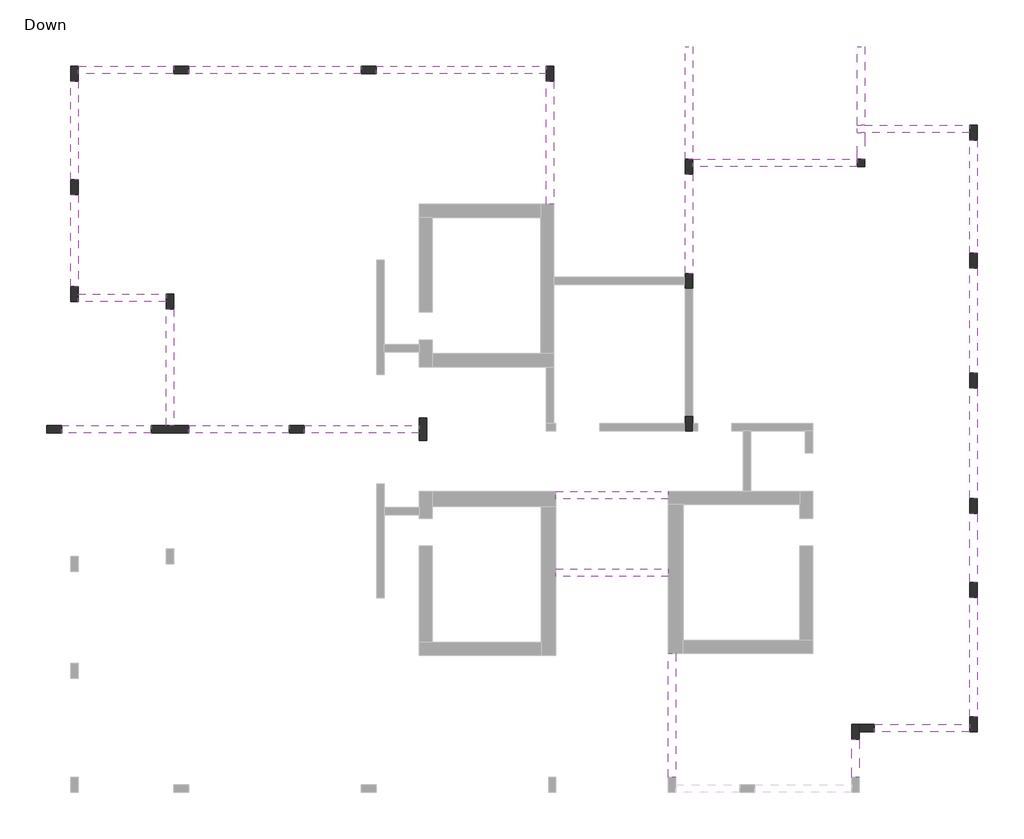
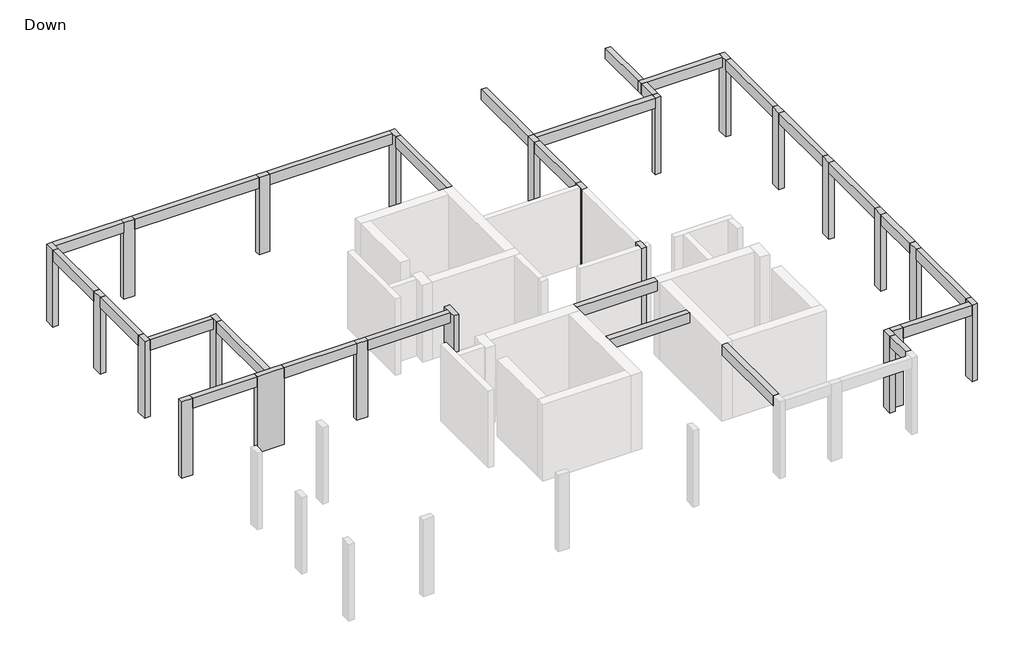
# One storey, part 2 of 2: 27 beams, 23 columns.
"""IFC4 building model written with IfcOpenShell, lengths in millimetres."""

from ifc_helpers import new_model, si_unit, frame, origin, origin_with_axes, place, context, project, spatial, polyline, outline, extrude, faceted_brep, element, save

model = new_model("IFC4")

# Units and contexts
model_context = context("Model", 3, world=origin())
ifc_project = project(units=[si_unit("LENGTHUNIT", "METRE", prefix="MILLI")], contexts=[model_context])

# Site, building, storey
site = spatial("IfcSite", under=ifc_project)
building = spatial("IfcBuilding", under=site)
storey = spatial("IfcBuildingStorey", under=building, Name="Down", Elevation=0.0)

# Beams
placement = place(None, origin())
element("IfcBeam", 1, ObjectType="Concrete Rectengular Beam : 20/40", at=placement, inside=storey, context=model_context, shape_type="SweptSolid", body=[
    extrude(outline(polyline([(-8952.4882749, 10699.8774677), (-8952.4882749, 10899.8774677), (-4346.8056177, 10899.8774677), (-4346.8056177, 10699.8774677), (-8952.4882749, 10699.8774677)])), frame((0.0, 0.0, 2600.0), z_axis=(0.0, 0.0, 1.0), x_axis=(1.0, 0.0, 0.0)), (0.0, 0.0, 1.0), 400.0),
])
element("IfcBeam", 2, ObjectType="Concrete Rectengular Beam : 20/40", at=placement, inside=storey, context=model_context, shape_type="Brep", body=[
    faceted_brep([(-11896.6244933, 10899.8774677, 3000.0), (-11896.6244933, 10699.8774677, 3000.0), (-9352.4882749, 10699.8774677, 3000.0), (-9352.4882749, 10899.8774677, 3000.0), (-11896.6244933, 10899.8774677, 2600.0), (-9352.4882749, 10899.8774677, 2600.0), (-11896.6244933, 10699.8774677, 2600.0), (-9352.4882749, 10699.8774677, 2600.0), (-11896.6244933, 10699.8774677, 2780.0)], [[[0, 1, 2, 3]], [[4, 0, 3, 5]], [[6, 4, 5, 7]], [[1, 8, 6, 7, 2]], [[1, 0, 4, 6, 8]], [[3, 2, 7, 5]]]),
])
element("IfcBeam", 3, ObjectType="Concrete Rectengular Beam : 20/40", at=placement, inside=storey, context=model_context, shape_type="SweptSolid", body=[
    extrude(outline(polyline([(-12096.6244933, 10499.8774677), (-11896.6244933, 10499.8774677), (-11896.6244933, 7862.3669988), (-12096.6244933, 7862.3669988), (-12096.6244933, 10499.8774677)])), frame((0.0, 0.0, 2600.0), z_axis=(0.0, 0.0, 1.0), x_axis=(1.0, 0.0, 0.0)), (0.0, 0.0, 1.0), 400.0),
])
element("IfcBeam", 4, ObjectType="Concrete Rectengular Beam : 20/40", at=placement, inside=storey, context=model_context, shape_type="SweptSolid", body=[
    extrude(outline(polyline([(-12096.6244933, 7462.3669988), (-11896.6244933, 7462.3669988), (-11896.6244933, 5012.2302086), (-12096.6244933, 5012.2302086), (-12096.6244933, 7462.3669988)])), frame((0.0, 0.0, 2600.0), z_axis=(0.0, 0.0, 1.0), x_axis=(1.0, 0.0, 0.0)), (0.0, 0.0, 1.0), 400.0),
])
element("IfcBeam", 5, ObjectType="Concrete Rectengular Beam : 20/40", at=placement, inside=storey, context=model_context, shape_type="Brep", body=[
    faceted_brep([(-9554.6843469, 4790.1128337, 3000.0), (-11896.6244933, 4790.1128337, 3000.0), (-11896.6244933, 4612.2302086, 3000.0), (-9554.6843469, 4612.2302086, 3000.0), (-9554.6843469, 4812.2302086, 2780.0), (-9554.6843469, 4812.2302086, 2600.0), (-11896.6244933, 4812.2302086, 2600.0), (-11896.6244933, 4812.2302086, 2780.0), (-9554.6843469, 4612.2302086, 2600.0), (-11896.6244933, 4612.2302086, 2600.0), (-9554.6843469, 4612.2302086, 2780.0), (-9554.6843469, 4790.1128337, 2780.0), (-11896.6244933, 4790.1128337, 2780.0)], [[[0, 1, 2, 3]], [[4, 5, 6, 7]], [[5, 8, 9, 6]], [[8, 10, 3, 2, 9]], [[8, 5, 4, 11, 0, 3, 10]], [[12, 11, 4, 7]], [[11, 12, 1, 0]], [[2, 1, 12, 7, 6, 9]]]),
])
element("IfcBeam", 6, ObjectType="Concrete Rectengular Beam : 20/40", at=placement, inside=storey, context=model_context, shape_type="Brep", body=[
    faceted_brep([(-9354.6843469, 4412.2302086, 3000.0), (-9554.6843469, 4412.2302086, 3000.0), (-9554.6843469, 1306.8737687, 3000.0), (-9354.6843469, 1306.8737687, 3000.0), (-9554.6843469, 4412.2302086, 2600.0), (-9554.6843469, 1306.8737687, 2600.0), (-9554.6843469, 1306.8737687, 2780.0), (-9354.6843469, 4412.2302086, 2600.0), (-9354.6843469, 1306.8737687, 2600.0), (-9354.6843469, 1306.8737687, 2780.0), (-9354.6843469, 4412.2302086, 2780.0)], [[[0, 1, 2, 3]], [[1, 4, 5, 6, 2]], [[4, 7, 8, 5]], [[0, 3, 9, 8, 7, 10]], [[1, 0, 10, 7, 4]], [[3, 2, 6, 5, 8, 9]]]),
])
element("IfcBeam", 7, ObjectType="Concrete Rectengular Beam : 20/40", at=placement, inside=storey, context=model_context, shape_type="SweptSolid", body=[
    extrude(outline(polyline([(-12343.1090323, 1106.8737687), (-12343.1090323, 1306.8737687), (-9954.6843469, 1306.8737687), (-9954.6843469, 1106.8737687), (-12343.1090323, 1106.8737687)])), frame((0.0, 0.0, 2600.0), z_axis=(0.0, 0.0, 1.0), x_axis=(1.0, 0.0, 0.0)), (0.0, 0.0, 1.0), 400.0),
])
element("IfcBeam", 8, ObjectType="Concrete Rectengular Beam : 20/40", at=placement, inside=storey, context=model_context, shape_type="SweptSolid", body=[
    extrude(outline(polyline([(-6260.2213409, 1306.8737687), (-6260.2213409, 1106.8737687), (-8954.6843469, 1106.8737687), (-8954.6843469, 1306.8737687), (-6260.2213409, 1306.8737687)])), frame((0.0, 0.0, 2600.0), z_axis=(0.0, 0.0, 1.0), x_axis=(1.0, 0.0, 0.0)), (0.0, 0.0, 1.0), 400.0),
])
element("IfcBeam", 9, ObjectType="Concrete Rectengular Beam : 20/40", at=placement, inside=storey, context=model_context, shape_type="Brep", body=[
    faceted_brep([(-5860.2213409, 1306.8737687, 3000.0), (-5860.2213409, 1106.8737687, 3000.0), (-2800.2213409, 1106.8737687, 3000.0), (-2800.2213409, 1306.8737687, 3000.0), (-5860.2213409, 1106.8737687, 2600.0), (-2800.2213409, 1106.8737687, 2600.0), (-2800.2213409, 1106.8737687, 2780.0), (-5860.2213409, 1306.8737687, 2600.0), (-2800.2213409, 1306.8737687, 2600.0), (-2800.2213409, 1306.8737687, 2780.0)], [[[0, 1, 2, 3]], [[1, 4, 5, 6, 2]], [[4, 7, 8, 5]], [[7, 0, 3, 9, 8]], [[1, 0, 7, 4]], [[3, 2, 6, 5, 8, 9]]]),
])
element("IfcBeam", 10, ObjectType="Concrete Rectengular Beam : 20/40", at=placement, inside=storey, context=model_context, shape_type="Brep", body=[
    faceted_brep([(-3946.8056177, 10899.8774677, 3000.0), (-3946.8056177, 10699.8774677, 3000.0), (592.5229388, 10699.8774677, 3000.0), (592.5229388, 10899.8774677, 3000.0), (-3946.8056177, 10699.8774677, 2600.0), (592.5229388, 10699.8774677, 2600.0), (592.5229388, 10699.8774677, 2780.0), (-3946.8056177, 10899.8774677, 2600.0), (592.5229388, 10899.8774677, 2600.0)], [[[0, 1, 2, 3]], [[1, 4, 5, 6, 2]], [[4, 7, 8, 5]], [[7, 0, 3, 8]], [[1, 0, 7, 4]], [[3, 2, 6, 5, 8]]]),
])
element("IfcBeam", 11, ObjectType="Concrete Rectengular Beam : 20/40", at=placement, inside=storey, context=model_context, shape_type="Brep", body=[
    faceted_brep([(792.5229388, 10499.8774677, 3000.0), (592.5229388, 10499.8774677, 3000.0), (592.5229388, 7208.2359353, 3000.0), (792.5229388, 7208.2359353, 3000.0), (592.5229388, 10499.8774677, 2600.0), (592.5229388, 7208.2359353, 2600.0), (592.5229388, 7208.2359353, 2780.0), (792.5229388, 10499.8774677, 2600.0), (792.5229388, 7208.2359353, 2600.0)], [[[0, 1, 2, 3]], [[1, 4, 5, 6, 2]], [[4, 7, 8, 5]], [[7, 0, 3, 8]], [[1, 0, 7, 4]], [[3, 2, 6, 5, 8]]]),
])
element("IfcBeam", 12, ObjectType="Concrete Rectengular Beam : 20/40", at=placement, inside=storey, context=model_context, shape_type="Brep", body=[
    faceted_brep([(4297.0462143, 5364.8955051, 3000.0), (4497.0462143, 5364.8955051, 3000.0), (4497.0462143, 8011.9737794, 3000.0), (4297.0462143, 8011.9737794, 3000.0), (4497.0462143, 5364.8955051, 2780.0), (4497.0462143, 5364.8955051, 2600.0), (4497.0462143, 8011.9737794, 2600.0), (4497.0462143, 8011.9737794, 2780.0), (4297.0462143, 5364.8955051, 2600.0), (4297.0462143, 8011.9737794, 2600.0)], [[[0, 1, 2, 3]], [[2, 1, 4, 5, 6, 7]], [[5, 8, 9, 6]], [[8, 0, 3, 9]], [[1, 0, 8, 5, 4]], [[3, 2, 7, 6, 9]]]),
])
element("IfcBeam", 13, ObjectType="Concrete Rectengular Beam : 20/40", at=placement, inside=storey, context=model_context, shape_type="Brep", body=[
    faceted_brep([(8746.3765637, -8086.1299304, 3000.0), (8946.3765637, -8086.1299304, 3000.0), (8946.3765637, -7081.7453909, 3000.0), (8746.3765637, -7081.7453909, 3000.0), (8946.3765637, -8086.1299304, 2600.0), (8946.3765637, -7081.7453909, 2600.0), (8746.3765637, -8086.1299304, 2600.0), (8746.3765637, -7081.7453909, 2600.0), (8746.3765637, -7081.7453909, 2780.0), (8746.3765637, -8086.1299304, 2780.0)], [[[0, 1, 2, 3]], [[1, 4, 5, 2]], [[4, 6, 7, 5]], [[0, 3, 8, 7, 6, 9]], [[1, 0, 9, 6, 4]], [[3, 2, 5, 7, 8]]]),
])
element("IfcBeam", 14, ObjectType="Concrete Rectengular Beam : 20/40", at=placement, inside=storey, context=model_context, shape_type="Brep", body=[
    faceted_brep([(9346.3765637, -6681.7453909, 3000.0), (9346.3765637, -6881.7453909, 3000.0), (11900.0250654, -6881.7453909, 3000.0), (11900.0250654, -6681.7453909, 3000.0), (9346.3765637, -6881.7453909, 2600.0), (11900.0250654, -6881.7453909, 2600.0), (9346.3765637, -6681.7453909, 2600.0), (11900.0250654, -6681.7453909, 2600.0), (11900.0250654, -6681.7453909, 2780.0), (9346.3765637, -6681.7453909, 2780.0)], [[[0, 1, 2, 3]], [[1, 4, 5, 2]], [[4, 6, 7, 5]], [[0, 3, 8, 7, 6, 9]], [[1, 0, 9, 6, 4]], [[3, 2, 5, 7, 8]]]),
])
element("IfcBeam", 15, ObjectType="Concrete Rectengular Beam : 20/40", at=placement, inside=storey, context=model_context, shape_type="Brep", body=[
    faceted_brep([(3852.6741008, -8086.1299304, 3000.0), (4052.6741008, -8086.1299304, 3000.0), (4052.6741008, -4782.6671723, 3000.0), (3852.6741008, -4782.6671723, 3000.0), (4052.6741008, -8086.1299304, 2600.0), (4052.6741008, -4782.6671723, 2600.0), (4052.6741008, -4782.6671723, 2780.0), (3852.6741008, -8086.1299304, 2600.0), (3852.6741008, -4782.6671723, 2600.0)], [[[0, 1, 2, 3]], [[1, 4, 5, 6, 2]], [[4, 7, 8, 5]], [[7, 0, 3, 8]], [[1, 0, 7, 4]], [[3, 2, 6, 5, 8]]]),
])
element("IfcBeam", 16, ObjectType="Concrete Rectengular Beam : 20/40", at=placement, inside=storey, context=model_context, shape_type="SweptSolid", body=[
    extrude(outline(polyline([(12100.0250654, -6481.7453909), (11900.0250654, -6481.7453909), (11900.0250654, -3292.2632704), (12100.0250654, -3292.2632704), (12100.0250654, -6481.7453909)])), frame((0.0, 0.0, 2600.0), z_axis=(0.0, 0.0, 1.0), x_axis=(1.0, 0.0, 0.0)), (0.0, 0.0, 1.0), 400.0),
])
element("IfcBeam", 17, ObjectType="Concrete Rectengular Beam : 20/40", at=placement, inside=storey, context=model_context, shape_type="SweptSolid", body=[
    extrude(outline(polyline([(12100.0250654, -2892.2632704), (11900.0250654, -2892.2632704), (11900.0250654, -1042.5387376), (12100.0250654, -1042.5387376), (12100.0250654, -2892.2632704)])), frame((0.0, 0.0, 2600.0), z_axis=(0.0, 0.0, 1.0), x_axis=(1.0, 0.0, 0.0)), (0.0, 0.0, 1.0), 400.0),
])
element("IfcBeam", 18, ObjectType="Concrete Rectengular Beam : 20/40", at=placement, inside=storey, context=model_context, shape_type="SweptSolid", body=[
    extrude(outline(polyline([(12100.0250654, -642.5387376), (11900.0250654, -642.5387376), (11900.0250654, 2306.6846493), (12100.0250654, 2306.6846493), (12100.0250654, -642.5387376)])), frame((0.0, 0.0, 2600.0), z_axis=(0.0, 0.0, 1.0), x_axis=(1.0, 0.0, 0.0)), (0.0, 0.0, 1.0), 400.0),
])
element("IfcBeam", 19, ObjectType="Concrete Rectengular Beam : 20/40", at=placement, inside=storey, context=model_context, shape_type="SweptSolid", body=[
    extrude(outline(polyline([(12100.0250654, 2706.6846493), (11900.0250654, 2706.6846493), (11900.0250654, 5508.9593048), (12100.0250654, 5508.9593048), (12100.0250654, 2706.6846493)])), frame((0.0, 0.0, 2600.0), z_axis=(0.0, 0.0, 1.0), x_axis=(1.0, 0.0, 0.0)), (0.0, 0.0, 1.0), 400.0),
])
element("IfcBeam", 20, ObjectType="Concrete Rectengular Beam : 20/40", at=placement, inside=storey, context=model_context, shape_type="SweptSolid", body=[
    extrude(outline(polyline([(12100.0250654, 5908.9593048), (11900.0250654, 5908.9593048), (11900.0250654, 8922.6036006), (12100.0250654, 8922.6036006), (12100.0250654, 5908.9593048)])), frame((0.0, 0.0, 2600.0), z_axis=(0.0, 0.0, 1.0), x_axis=(1.0, 0.0, 0.0)), (0.0, 0.0, 1.0), 400.0),
])
element("IfcBeam", 21, ObjectType="Concrete Rectengular Beam : 20/40", at=placement, inside=storey, context=model_context, shape_type="Brep", body=[
    faceted_brep([(8895.1583714, 8211.9737794, 3000.0), (8895.1583714, 8411.9737794, 3000.0), (4497.0462143, 8411.9737794, 3000.0), (4497.0462143, 8211.9737794, 3000.0), (8895.1583714, 8411.9737794, 2780.0), (8895.1583714, 8411.9737794, 2600.0), (4497.0462143, 8411.9737794, 2600.0), (4497.0462143, 8411.9737794, 2780.0), (8895.1583714, 8211.9737794, 2600.0), (4497.0462143, 8211.9737794, 2600.0), (4497.0462143, 8211.9737794, 2780.0), (8895.1583714, 8211.9737794, 2780.0)], [[[0, 1, 2, 3]], [[1, 4, 5, 6, 7, 2]], [[5, 8, 9, 6]], [[0, 3, 10, 9, 8, 11]], [[3, 2, 7, 6, 9, 10]], [[1, 0, 11, 8, 5, 4]]]),
])
element("IfcBeam", 22, ObjectType="Concrete Rectengular Beam : 20/40", at=placement, inside=storey, context=model_context, shape_type="Brep", body=[
    faceted_brep([(8895.1583714, 9322.6036006, 3000.0), (8895.1583714, 9122.6036006, 3000.0), (9095.1583714, 9122.6036006, 3000.0), (11900.0250654, 9122.6036006, 3000.0), (11900.0250654, 9322.6036006, 3000.0), (9095.1583714, 9322.6036006, 3000.0), (8895.1583714, 9122.6036006, 2600.0), (9095.1583714, 9122.6036006, 2600.0), (11900.0250654, 9122.6036006, 2600.0), (11900.0250654, 9122.6036006, 2780.0), (8895.1583714, 9322.6036006, 2600.0), (9095.1583714, 9322.6036006, 2600.0), (11900.0250654, 9322.6036006, 2600.0)], [[[0, 1, 2, 3, 4, 5]], [[1, 6, 7, 8, 9, 3, 2]], [[6, 10, 11, 12, 8, 7]], [[10, 0, 5, 4, 12, 11]], [[4, 3, 9, 8, 12]], [[1, 0, 10, 6]]]),
])
element("IfcBeam", 23, ObjectType="Concrete Rectengular Beam : 20/40", at=placement, inside=storey, context=model_context, shape_type="Brep", body=[
    faceted_brep([(8895.1583714, 8411.9737794, 3000.0), (9095.1583714, 8411.9737794, 3000.0), (9095.1583714, 9122.6036006, 3000.0), (8895.1583714, 9122.6036006, 3000.0), (9095.1583714, 8411.9737794, 2780.0), (9095.1583714, 8411.9737794, 2600.0), (9095.1583714, 9122.6036006, 2600.0), (9095.1583714, 9122.6036006, 2780.0), (8895.1583714, 8411.9737794, 2600.0), (8895.1583714, 9122.6036006, 2600.0), (8895.1583714, 8411.9737794, 2780.0)], [[[0, 1, 2, 3]], [[2, 1, 4, 5, 6, 7]], [[5, 8, 9, 6]], [[8, 10, 0, 3, 9]], [[0, 10, 8, 5, 4, 1]], [[3, 2, 7, 6, 9]]]),
])
element("IfcBeam", 24, ObjectType="Concrete Rectengular Beam : 20/40", at=placement, inside=storey, context=model_context, shape_type="Brep", body=[
    faceted_brep([(4297.0462143, 11422.6036006, 3000.0), (4497.0462143, 11422.6036006, 3000.0), (4497.0462143, 11422.6036006, 2780.0), (4497.0462143, 11422.6036006, 2600.0), (4297.0462143, 11422.6036006, 2600.0), (4297.0462143, 8411.9737794, 3000.0), (4497.0462143, 8411.9737794, 3000.0), (4497.0462143, 8411.9737794, 2780.0), (4497.0462143, 8411.9737794, 2600.0), (4297.0462143, 8411.9737794, 2600.0)], [[[0, 1, 2, 3, 4]], [[1, 0, 5, 6]], [[3, 2, 1, 6, 7, 8]], [[4, 3, 8, 9]], [[0, 4, 9, 5]], [[8, 7, 6, 5, 9]]]),
])
element("IfcBeam", 25, ObjectType="Concrete Rectengular Beam : 20/40", at=placement, inside=storey, context=model_context, shape_type="Brep", body=[
    faceted_brep([(8895.1583714, 11422.6036006, 3000.0), (9095.1583714, 11422.6036006, 3000.0), (9095.1583714, 11422.6036006, 2600.0), (8895.1583714, 11422.6036006, 2600.0), (8895.1583714, 11422.6036006, 2780.0), (8895.1583714, 9322.6036006, 3000.0), (9095.1583714, 9322.6036006, 3000.0), (9095.1583714, 9322.6036006, 2600.0), (8895.1583714, 9322.6036006, 2600.0)], [[[0, 1, 2, 3, 4]], [[1, 0, 5, 6]], [[2, 1, 6, 7]], [[3, 2, 7, 8]], [[0, 4, 3, 8, 5]], [[6, 5, 8, 7]]]),
])
element("IfcBeam", 26, ObjectType="Concrete Rectengular Beam : 20/40", at=placement, inside=storey, context=model_context, shape_type="SweptSolid", body=[
    extrude(outline(polyline([(852.6741008, -654.488398), (852.6741008, -454.488398), (3852.6741008, -454.488398), (3852.6741008, -654.488398), (852.6741008, -654.488398)])), frame((0.0, 0.0, 2600.0), z_axis=(0.0, 0.0, 1.0), x_axis=(1.0, 0.0, 0.0)), (0.0, 0.0, 1.0), 400.0),
])
element("IfcBeam", 27, ObjectType="Concrete Rectengular Beam : 20/40", at=placement, inside=storey, context=model_context, shape_type="SweptSolid", body=[
    extrude(outline(polyline([(852.6741008, -2731.143802), (852.6741008, -2531.143802), (3852.6741008, -2531.143802), (3852.6741008, -2731.143802), (852.6741008, -2731.143802)])), frame((0.0, 0.0, 2600.0), z_axis=(0.0, 0.0, 1.0), x_axis=(1.0, 0.0, 0.0)), (0.0, 0.0, 1.0), 400.0),
])

# Columns
element("IfcColumn", 28, ObjectType="Concrete Rectengular Column : 20/100", at=placement, inside=storey, context=model_context, shape_type="Brep", body=[
    faceted_brep([(-9954.6843469, 1306.8737687, 0.0), (-8954.6843469, 1306.8737687, 0.0), (-8954.6843469, 1106.8737687, 0.0), (-9954.6843469, 1106.8737687, 0.0), (-9954.6843469, 1306.8737687, 3000.0), (-9554.6843469, 1306.8737687, 3000.0), (-9354.6843469, 1306.8737687, 3000.0), (-8954.6843469, 1306.8737687, 3000.0), (-8954.6843469, 1106.8737687, 3000.0), (-9354.6843469, 1106.8737687, 3000.0), (-9554.6843469, 1106.8737687, 3000.0), (-9954.6843469, 1106.8737687, 3000.0)], [[[0, 1, 2, 3]], [[4, 5, 6, 7, 1, 0]], [[7, 8, 2, 1]], [[8, 9, 10, 11, 3, 2]], [[11, 4, 0, 3]], [[4, 11, 10, 9, 8, 7, 6, 5]]]),
])
element("IfcColumn", 29, ObjectType="Concrete Rectengular Column : 20/20", at=placement, inside=storey, context=model_context, shape_type="Brep", body=[
    faceted_brep([(9095.1583714, 8411.9737794, 0.0), (9095.1583714, 8211.9737794, 0.0), (8895.1583714, 8211.9737794, 0.0), (8895.1583714, 8411.9737794, 0.0), (9095.1583714, 8411.9737794, 3000.0), (9095.1583714, 8211.9737794, 3000.0), (9095.1583714, 8211.9737794, 2780.0), (8895.1583714, 8211.9737794, 3000.0), (8895.1583714, 8411.9737794, 3000.0)], [[[0, 1, 2, 3]], [[4, 5, 6, 1, 0]], [[5, 7, 2, 1, 6]], [[7, 8, 3, 2]], [[8, 4, 0, 3]], [[4, 8, 7, 5]]]),
])
element("IfcColumn", 30, ObjectType="Concrete Rectengular Column : 20/40", at=placement, inside=storey, context=model_context, shape_type="Brep", body=[
    faceted_brep([(-11896.6244933, 10899.8774677, 0.0), (-11896.6244933, 10499.8774677, 0.0), (-12096.6244933, 10499.8774677, 0.0), (-12096.6244933, 10899.8774677, 0.0), (-11896.6244933, 10899.8774677, 3000.0), (-11896.6244933, 10699.8774677, 3000.0), (-11896.6244933, 10499.8774677, 3000.0), (-12096.6244933, 10499.8774677, 3000.0), (-12096.6244933, 10899.8774677, 3000.0)], [[[0, 1, 2, 3]], [[4, 5, 6, 1, 0]], [[6, 7, 2, 1]], [[7, 8, 3, 2]], [[8, 4, 0, 3]], [[4, 8, 7, 6, 5]]]),
])
element("IfcColumn", 31, ObjectType="Concrete Rectengular Column : 20/40", at=placement, inside=storey, context=model_context, shape_type="SweptSolid", body=[
    extrude(outline(polyline([(-9352.4882749, 10899.8774677), (-8952.4882749, 10899.8774677), (-8952.4882749, 10699.8774677), (-9352.4882749, 10699.8774677), (-9352.4882749, 10899.8774677)])), origin_with_axes(), (0.0, 0.0, 1.0), 3000.0),
])
element("IfcColumn", 32, ObjectType="Concrete Rectengular Column : 20/40", at=placement, inside=storey, context=model_context, shape_type="SweptSolid", body=[
    extrude(outline(polyline([(-4346.8056177, 10899.8774677), (-3946.8056177, 10899.8774677), (-3946.8056177, 10699.8774677), (-4346.8056177, 10699.8774677), (-4346.8056177, 10899.8774677)])), origin_with_axes(), (0.0, 0.0, 1.0), 3000.0),
])
element("IfcColumn", 33, ObjectType="Concrete Rectengular Column : 20/40", at=placement, inside=storey, context=model_context, shape_type="Brep", body=[
    faceted_brep([(592.5229388, 10499.8774677, 0.0), (592.5229388, 10899.8774677, 0.0), (792.5229388, 10899.8774677, 0.0), (792.5229388, 10499.8774677, 0.0), (592.5229388, 10499.8774677, 3000.0), (592.5229388, 10699.8774677, 3000.0), (592.5229388, 10899.8774677, 3000.0), (792.5229388, 10899.8774677, 3000.0), (792.5229388, 10499.8774677, 3000.0)], [[[0, 1, 2, 3]], [[4, 5, 6, 1, 0]], [[6, 7, 2, 1]], [[7, 8, 3, 2]], [[8, 4, 0, 3]], [[4, 8, 7, 6, 5]]]),
])
element("IfcColumn", 34, ObjectType="Concrete Rectengular Column : 20/40", at=placement, inside=storey, context=model_context, shape_type="SweptSolid", body=[
    extrude(outline(polyline([(-12096.6244933, 7462.3669988), (-12096.6244933, 7862.3669988), (-11896.6244933, 7862.3669988), (-11896.6244933, 7462.3669988), (-12096.6244933, 7462.3669988)])), origin_with_axes(), (0.0, 0.0, 1.0), 3000.0),
])
element("IfcColumn", 35, ObjectType="Concrete Rectengular Column : 20/40", at=placement, inside=storey, context=model_context, shape_type="Brep", body=[
    faceted_brep([(-12096.6244933, 4612.2302086, 0.0), (-12096.6244933, 5012.2302086, 0.0), (-11896.6244933, 5012.2302086, 0.0), (-11896.6244933, 4612.2302086, 0.0), (-12096.6244933, 4612.2302086, 3000.0), (-12096.6244933, 5012.2302086, 3000.0), (-11896.6244933, 5012.2302086, 3000.0), (-11896.6244933, 4790.1128337, 3000.0), (-11896.6244933, 4612.2302086, 3000.0)], [[[0, 1, 2, 3]], [[4, 5, 1, 0]], [[5, 6, 2, 1]], [[6, 7, 8, 3, 2]], [[8, 4, 0, 3]], [[4, 8, 7, 6, 5]]]),
])
element("IfcColumn", 36, ObjectType="Concrete Rectengular Column : 20/40", at=placement, inside=storey, context=model_context, shape_type="Brep", body=[
    faceted_brep([(-9554.6843469, 4412.2302086, 0.0), (-9554.6843469, 4812.2302086, 0.0), (-9354.6843469, 4812.2302086, 0.0), (-9354.6843469, 4412.2302086, 0.0), (-9554.6843469, 4412.2302086, 3000.0), (-9554.6843469, 4612.2302086, 3000.0), (-9554.6843469, 4790.1128337, 3000.0), (-9554.6843469, 4812.2302086, 3000.0), (-9554.6843469, 4812.2302086, 2780.0), (-9354.6843469, 4812.2302086, 3000.0), (-9354.6843469, 4812.2302086, 2780.0), (-9354.6843469, 4412.2302086, 3000.0)], [[[0, 1, 2, 3]], [[4, 5, 6, 7, 8, 1, 0]], [[7, 9, 10, 2, 1, 8]], [[9, 11, 3, 2, 10]], [[11, 4, 0, 3]], [[4, 11, 9, 7, 6, 5]]]),
])
element("IfcColumn", 37, ObjectType="Concrete Rectengular Column : 20/40", at=placement, inside=storey, context=model_context, shape_type="Brep", body=[
    faceted_brep([(-12343.1090323, 1106.8737687, 0.0), (-12743.1090323, 1106.8737687, 0.0), (-12743.1090323, 1306.8737687, 0.0), (-12343.1090323, 1306.8737687, 0.0), (-12343.1090323, 1106.8737687, 3000.0), (-12743.1090323, 1106.8737687, 3000.0), (-12743.1090323, 1106.8737687, 2780.0), (-12743.1090323, 1306.8737687, 3000.0), (-12743.1090323, 1306.8737687, 2780.0), (-12343.1090323, 1306.8737687, 3000.0)], [[[0, 1, 2, 3]], [[4, 5, 6, 1, 0]], [[5, 7, 8, 2, 1, 6]], [[7, 9, 3, 2, 8]], [[9, 4, 0, 3]], [[4, 9, 7, 5]]]),
])
element("IfcColumn", 38, ObjectType="Concrete Rectengular Column : 20/40", at=placement, inside=storey, context=model_context, shape_type="SweptSolid", body=[
    extrude(outline(polyline([(-5860.2213409, 1106.8737687), (-6260.2213409, 1106.8737687), (-6260.2213409, 1306.8737687), (-5860.2213409, 1306.8737687), (-5860.2213409, 1106.8737687)])), origin_with_axes(), (0.0, 0.0, 1.0), 3000.0),
])
element("IfcColumn", 39, ObjectType="Concrete Rectengular Column : 20/40", at=placement, inside=storey, context=model_context, shape_type="Brep", body=[
    faceted_brep([(8746.3765637, -7081.7453909, 0.0), (8746.3765637, -6681.7453909, 0.0), (8946.3765637, -6681.7453909, 0.0), (8946.3765637, -6881.7453909, 0.0), (8946.3765637, -7081.7453909, 0.0), (8746.3765637, -7081.7453909, 3000.0), (8746.3765637, -6681.7453909, 3000.0), (8746.3765637, -6681.7453909, 2780.0), (8946.3765637, -6681.7453909, 3000.0), (8946.3765637, -6881.7453909, 3000.0), (8946.3765637, -7081.7453909, 3000.0)], [[[0, 1, 2, 3, 4]], [[5, 6, 7, 1, 0]], [[6, 8, 2, 1, 7]], [[8, 9, 10, 4, 3, 2]], [[10, 5, 0, 4]], [[5, 10, 9, 8, 6]]]),
])
element("IfcColumn", 40, ObjectType="Concrete Rectengular Column : 20/40", at=placement, inside=storey, context=model_context, shape_type="SweptSolid", body=[
    extrude(outline(polyline([(9346.3765637, -6881.7453909), (8946.3765637, -6881.7453909), (8946.3765637, -6681.7453909), (9346.3765637, -6681.7453909), (9346.3765637, -6881.7453909)])), origin_with_axes(), (0.0, 0.0, 1.0), 3000.0),
])
element("IfcColumn", 41, ObjectType="Concrete Rectengular Column : 20/40", at=placement, inside=storey, context=model_context, shape_type="Brep", body=[
    faceted_brep([(12100.0250654, -6481.7453909, 0.0), (12100.0250654, -6881.7453909, 0.0), (11900.0250654, -6881.7453909, 0.0), (11900.0250654, -6481.7453909, 0.0), (12100.0250654, -6481.7453909, 3000.0), (12100.0250654, -6881.7453909, 3000.0), (11900.0250654, -6881.7453909, 3000.0), (11900.0250654, -6681.7453909, 3000.0), (11900.0250654, -6481.7453909, 3000.0)], [[[0, 1, 2, 3]], [[4, 5, 1, 0]], [[5, 6, 2, 1]], [[6, 7, 8, 3, 2]], [[8, 4, 0, 3]], [[4, 8, 7, 6, 5]]]),
])
element("IfcColumn", 42, ObjectType="Concrete Rectengular Column : 20/40", at=placement, inside=storey, context=model_context, shape_type="SweptSolid", body=[
    extrude(outline(polyline([(12100.0250654, -2892.2632704), (12100.0250654, -3292.2632704), (11900.0250654, -3292.2632704), (11900.0250654, -2892.2632704), (12100.0250654, -2892.2632704)])), origin_with_axes(), (0.0, 0.0, 1.0), 3000.0),
])
element("IfcColumn", 43, ObjectType="Concrete Rectengular Column : 20/40", at=placement, inside=storey, context=model_context, shape_type="SweptSolid", body=[
    extrude(outline(polyline([(12100.0250654, -642.5387376), (12100.0250654, -1042.5387376), (11900.0250654, -1042.5387376), (11900.0250654, -642.5387376), (12100.0250654, -642.5387376)])), origin_with_axes(), (0.0, 0.0, 1.0), 3000.0),
])
element("IfcColumn", 44, ObjectType="Concrete Rectengular Column : 20/40", at=placement, inside=storey, context=model_context, shape_type="SweptSolid", body=[
    extrude(outline(polyline([(12100.0250654, 2706.6846493), (12100.0250654, 2306.6846493), (11900.0250654, 2306.6846493), (11900.0250654, 2706.6846493), (12100.0250654, 2706.6846493)])), origin_with_axes(), (0.0, 0.0, 1.0), 3000.0),
])
element("IfcColumn", 45, ObjectType="Concrete Rectengular Column : 20/40", at=placement, inside=storey, context=model_context, shape_type="SweptSolid", body=[
    extrude(outline(polyline([(12100.0250654, 5908.9593048), (12100.0250654, 5508.9593048), (11900.0250654, 5508.9593048), (11900.0250654, 5908.9593048), (12100.0250654, 5908.9593048)])), origin_with_axes(), (0.0, 0.0, 1.0), 3000.0),
])
element("IfcColumn", 46, ObjectType="Concrete Rectengular Column : 20/40", at=placement, inside=storey, context=model_context, shape_type="Brep", body=[
    faceted_brep([(12100.0250654, 9322.6036006, 0.0), (12100.0250654, 8922.6036006, 0.0), (11900.0250654, 8922.6036006, 0.0), (11900.0250654, 9322.6036006, 0.0), (12100.0250654, 9322.6036006, 3000.0), (12100.0250654, 8922.6036006, 3000.0), (11900.0250654, 8922.6036006, 3000.0), (11900.0250654, 9122.6036006, 3000.0), (11900.0250654, 9322.6036006, 3000.0)], [[[0, 1, 2, 3]], [[4, 5, 1, 0]], [[5, 6, 2, 1]], [[6, 7, 8, 3, 2]], [[8, 4, 0, 3]], [[4, 8, 7, 6, 5]]]),
])
element("IfcColumn", 47, ObjectType="Concrete Rectengular Column : 20/40", at=placement, inside=storey, context=model_context, shape_type="Brep", body=[
    faceted_brep([(4497.0462143, 1557.9050688, 0.0), (4497.0462143, 1357.9050688, 0.0), (4497.0462143, 1157.9050688, 0.0), (4297.0462143, 1157.9050688, 0.0), (4297.0462143, 1357.9050688, 0.0), (4297.0462143, 1557.9050688, 0.0), (4497.0462143, 1557.9050688, 3000.0), (4497.0462143, 1357.9050688, 3000.0), (4497.0462143, 1157.9050688, 3000.0), (4297.0462143, 1157.9050688, 3000.0), (4297.0462143, 1357.9050688, 3000.0), (4297.0462143, 1557.9050688, 3000.0)], [[[0, 1, 2, 3, 4, 5]], [[6, 7, 8, 2, 1, 0]], [[8, 9, 3, 2]], [[9, 10, 11, 5, 4, 3]], [[11, 6, 0, 5]], [[6, 11, 10, 9, 8, 7]]]),
])
element("IfcColumn", 48, ObjectType="Concrete Rectengular Column : 20/40", at=placement, inside=storey, context=model_context, shape_type="Brep", body=[
    faceted_brep([(4497.0462143, 5364.8955051, 0.0), (4497.0462143, 4964.8955051, 0.0), (4297.0462143, 4964.8955051, 0.0), (4297.0462143, 5064.8955051, 0.0), (4297.0462143, 5264.8955051, 0.0), (4297.0462143, 5364.8955051, 0.0), (4497.0462143, 5364.8955051, 3000.0), (4497.0462143, 4964.8955051, 3000.0), (4297.0462143, 4964.8955051, 3000.0), (4297.0462143, 5064.8955051, 3000.0), (4297.0462143, 5264.8955051, 3000.0), (4297.0462143, 5364.8955051, 3000.0)], [[[0, 1, 2, 3, 4, 5]], [[6, 7, 1, 0]], [[7, 8, 2, 1]], [[8, 9, 10, 11, 5, 4, 3, 2]], [[11, 6, 0, 5]], [[6, 11, 10, 9, 8, 7]]]),
])
element("IfcColumn", 49, ObjectType="Concrete Rectengular Column : 20/40", at=placement, inside=storey, context=model_context, shape_type="Brep", body=[
    faceted_brep([(4497.0462143, 8411.9737794, 0.0), (4497.0462143, 8011.9737794, 0.0), (4297.0462143, 8011.9737794, 0.0), (4297.0462143, 8411.9737794, 0.0), (4497.0462143, 8411.9737794, 3000.0), (4497.0462143, 8211.9737794, 3000.0), (4497.0462143, 8011.9737794, 3000.0), (4297.0462143, 8011.9737794, 3000.0), (4297.0462143, 8411.9737794, 3000.0)], [[[0, 1, 2, 3]], [[4, 5, 6, 1, 0]], [[6, 7, 2, 1]], [[7, 8, 3, 2]], [[8, 4, 0, 3]], [[4, 8, 7, 6, 5]]]),
])
element("IfcColumn", 50, ObjectType="Concrete Rectengular Column : 20/60", at=placement, inside=storey, context=model_context, shape_type="Brep", body=[
    faceted_brep([(-2600.2213409, 1506.8737687, 0.0), (-2600.2213409, 906.8737687, 0.0), (-2800.2213409, 906.8737687, 0.0), (-2800.2213409, 1506.8737687, 0.0), (-2600.2213409, 1506.8737687, 3000.0), (-2600.2213409, 906.8737687, 3000.0), (-2600.2213409, 906.8737687, 2780.0), (-2600.2213409, 1506.8737687, 2780.0), (-2800.2213409, 906.8737687, 3000.0), (-2800.2213409, 906.8737687, 2780.0), (-2800.2213409, 1106.8737687, 3000.0), (-2800.2213409, 1306.8737687, 3000.0), (-2800.2213409, 1506.8737687, 3000.0), (-2800.2213409, 1506.8737687, 2780.0)], [[[0, 1, 2, 3]], [[4, 5, 6, 1, 0, 7]], [[5, 8, 9, 2, 1, 6]], [[8, 10, 11, 12, 13, 3, 2, 9]], [[12, 4, 7, 0, 3, 13]], [[4, 12, 11, 10, 8, 5]]]),
])

save(model, "model.ifc")

# Revit data of these elements
# Type "Concrete Rectengular Beam : 20/40"
#   Keynote = "09000"
#   Length [instance default] = 152.4 cm
#   b = 20 cm
#   h = 40 cm
#   Structural Material [instance default] = Concrete
#   Assembly Code = ""
# Type "Concrete Rectengular Column : 20/100"
#   b = 20 cm
#   h = 100 cm
#   Structural Material [instance default] = Concrete
# Type "Concrete Rectengular Column : 20/20"
#   b = 20 cm
#   h = 20 cm
#   Structural Material [instance default] = Concrete
# Type "Concrete Rectengular Column : 20/40"
#   b = 20 cm
#   h = 40 cm
#   Structural Material [instance default] = Concrete
# Type "Concrete Rectengular Column : 20/60"
#   b = 20 cm
#   h = 60 cm
#   Structural Material [instance default] = Concrete
# Element 1 (IfcBeam, "Concrete Rectengular Beam : 20/40")
#   Comments = ""
#   Mark = "B1"
#   SOFiSTiK_AMG_Comments = ""
#   SOFiSTiK_AMG_Scheduled = yes
#   SOFiSTiK_AMG_Adjusted = yes
#   Structural Material = Concrete
#   Phase Created = New Construction
#   Materials on its faces: "Concrete"
# Element 2 (IfcBeam, "Concrete Rectengular Beam : 20/40")
#   Comments = ""
#   Mark = "B2"
#   SOFiSTiK_AMG_Comments = ""
#   SOFiSTiK_AMG_Scheduled = yes
#   SOFiSTiK_AMG_Adjusted = yes
#   Structural Material = Concrete
#   Phase Created = New Construction
#   Materials on its faces: "Concrete"
# Element 3 (IfcBeam, "Concrete Rectengular Beam : 20/40")
#   Comments = ""
#   Mark = "B3"
#   SOFiSTiK_AMG_Comments = ""
#   SOFiSTiK_AMG_Scheduled = yes
#   SOFiSTiK_AMG_Adjusted = yes
#   Structural Material = Concrete
#   Phase Created = New Construction
#   Materials on its faces: "Concrete"
# Element 4 (IfcBeam, "Concrete Rectengular Beam : 20/40")
#   Comments = ""
#   Mark = "B4"
#   SOFiSTiK_AMG_Comments = ""
#   SOFiSTiK_AMG_Scheduled = yes
#   SOFiSTiK_AMG_Adjusted = yes
#   Structural Material = Concrete
#   Phase Created = New Construction
#   Materials on its faces: "Concrete"
# Element 5 (IfcBeam, "Concrete Rectengular Beam : 20/40")
#   Comments = ""
#   Mark = "B5"
#   SOFiSTiK_AMG_Comments = ""
#   SOFiSTiK_AMG_Scheduled = yes
#   SOFiSTiK_AMG_Adjusted = yes
#   Structural Material = Concrete
#   Phase Created = New Construction
#   Materials on its faces: "Concrete"
# Element 6 (IfcBeam, "Concrete Rectengular Beam : 20/40")
#   Comments = ""
#   Mark = "B6"
#   SOFiSTiK_AMG_Comments = ""
#   SOFiSTiK_AMG_Scheduled = yes
#   SOFiSTiK_AMG_Adjusted = yes
#   Structural Material = Concrete
#   Phase Created = New Construction
#   Materials on its faces: "Concrete"
# Element 7 (IfcBeam, "Concrete Rectengular Beam : 20/40")
#   Comments = ""
#   Mark = "B7"
#   SOFiSTiK_AMG_Comments = ""
#   SOFiSTiK_AMG_Scheduled = yes
#   SOFiSTiK_AMG_Adjusted = yes
#   Structural Material = Concrete
#   Phase Created = New Construction
#   Materials on its faces: "Concrete"
# Element 8 (IfcBeam, "Concrete Rectengular Beam : 20/40")
#   Comments = ""
#   Mark = "B8"
#   SOFiSTiK_AMG_Comments = ""
#   SOFiSTiK_AMG_Scheduled = yes
#   SOFiSTiK_AMG_Adjusted = yes
#   Structural Material = Concrete
#   Phase Created = New Construction
#   Materials on its faces: "Concrete"
# Element 9 (IfcBeam, "Concrete Rectengular Beam : 20/40")
#   Comments = ""
#   Mark = "B9"
#   SOFiSTiK_AMG_Comments = ""
#   SOFiSTiK_AMG_Scheduled = yes
#   SOFiSTiK_AMG_Adjusted = yes
#   Structural Material = Concrete
#   Phase Created = New Construction
#   Materials on its faces: "Concrete"
# Element 10 (IfcBeam, "Concrete Rectengular Beam : 20/40")
#   Comments = ""
#   Mark = "B10"
#   SOFiSTiK_AMG_Comments = ""
#   SOFiSTiK_AMG_Scheduled = yes
#   SOFiSTiK_AMG_Adjusted = yes
#   Structural Material = Concrete
#   Phase Created = New Construction
#   Materials on its faces: "Concrete"
# Element 11 (IfcBeam, "Concrete Rectengular Beam : 20/40")
#   Comments = ""
#   Mark = "B11"
#   SOFiSTiK_AMG_Comments = ""
#   SOFiSTiK_AMG_Scheduled = yes
#   SOFiSTiK_AMG_Adjusted = yes
#   Structural Material = Concrete
#   Phase Created = New Construction
#   Materials on its faces: "Concrete"
# Element 12 (IfcBeam, "Concrete Rectengular Beam : 20/40")
#   Comments = ""
#   Mark = "B20"
#   SOFiSTiK_AMG_Comments = ""
#   SOFiSTiK_AMG_Scheduled = yes
#   SOFiSTiK_AMG_Adjusted = yes
#   Structural Material = Concrete
#   Phase Created = New Construction
#   Materials on its faces: "Concrete"
# Element 13 (IfcBeam, "Concrete Rectengular Beam : 20/40")
#   Comments = ""
#   Mark = "B23"
#   SOFiSTiK_AMG_Comments = ""
#   SOFiSTiK_AMG_Scheduled = yes
#   SOFiSTiK_AMG_Adjusted = yes
#   Structural Material = Concrete
#   Phase Created = New Construction
#   Materials on its faces: "Concrete"
# Element 14 (IfcBeam, "Concrete Rectengular Beam : 20/40")
#   Comments = ""
#   Mark = "B24"
#   SOFiSTiK_AMG_Comments = ""
#   SOFiSTiK_AMG_Scheduled = yes
#   SOFiSTiK_AMG_Adjusted = yes
#   Structural Material = Concrete
#   Phase Created = New Construction
#   Materials on its faces: "Concrete"
# Element 15 (IfcBeam, "Concrete Rectengular Beam : 20/40")
#   Comments = ""
#   Mark = "B25"
#   SOFiSTiK_AMG_Comments = ""
#   SOFiSTiK_AMG_Scheduled = yes
#   SOFiSTiK_AMG_Adjusted = yes
#   Structural Material = Concrete
#   Phase Created = New Construction
#   Materials on its faces: "Concrete"
# Element 16 (IfcBeam, "Concrete Rectengular Beam : 20/40")
#   Comments = ""
#   Mark = "B26"
#   SOFiSTiK_AMG_Comments = ""
#   SOFiSTiK_AMG_Scheduled = yes
#   SOFiSTiK_AMG_Adjusted = yes
#   Structural Material = Concrete
#   Phase Created = New Construction
#   Materials on its faces: "Concrete"
# Element 17 (IfcBeam, "Concrete Rectengular Beam : 20/40")
#   Comments = ""
#   Mark = "B27"
#   SOFiSTiK_AMG_Comments = ""
#   SOFiSTiK_AMG_Scheduled = yes
#   SOFiSTiK_AMG_Adjusted = yes
#   Structural Material = Concrete
#   Phase Created = New Construction
#   Materials on its faces: "Concrete"
# Element 18 (IfcBeam, "Concrete Rectengular Beam : 20/40")
#   Comments = ""
#   Mark = "B28"
#   SOFiSTiK_AMG_Comments = ""
#   SOFiSTiK_AMG_Scheduled = yes
#   SOFiSTiK_AMG_Adjusted = yes
#   Structural Material = Concrete
#   Phase Created = New Construction
#   Materials on its faces: "Concrete"
# Element 19 (IfcBeam, "Concrete Rectengular Beam : 20/40")
#   Comments = ""
#   Mark = "B29"
#   SOFiSTiK_AMG_Comments = ""
#   SOFiSTiK_AMG_Scheduled = yes
#   SOFiSTiK_AMG_Adjusted = yes
#   Structural Material = Concrete
#   Phase Created = New Construction
#   Materials on its faces: "Concrete"
# Element 20 (IfcBeam, "Concrete Rectengular Beam : 20/40")
#   Comments = ""
#   Mark = "B30"
#   SOFiSTiK_AMG_Comments = ""
#   SOFiSTiK_AMG_Scheduled = yes
#   SOFiSTiK_AMG_Adjusted = yes
#   Structural Material = Concrete
#   Phase Created = New Construction
#   Materials on its faces: "Concrete"
# Element 21 (IfcBeam, "Concrete Rectengular Beam : 20/40")
#   Comments = ""
#   Mark = "B31"
#   SOFiSTiK_AMG_Comments = ""
#   SOFiSTiK_AMG_Scheduled = yes
#   SOFiSTiK_AMG_Adjusted = yes
#   Structural Material = Concrete
#   Phase Created = New Construction
#   Materials on its faces: "Concrete"
# Element 22 (IfcBeam, "Concrete Rectengular Beam : 20/40")
#   Comments = ""
#   Mark = "B32"
#   SOFiSTiK_AMG_Comments = ""
#   SOFiSTiK_AMG_Scheduled = yes
#   SOFiSTiK_AMG_Adjusted = yes
#   Structural Material = Concrete
#   Phase Created = New Construction
#   Materials on its faces: "Concrete"
# Element 23 (IfcBeam, "Concrete Rectengular Beam : 20/40")
#   Comments = ""
#   Mark = "B33"
#   SOFiSTiK_AMG_Comments = ""
#   SOFiSTiK_AMG_Scheduled = yes
#   SOFiSTiK_AMG_Adjusted = yes
#   Structural Material = Concrete
#   Phase Created = New Construction
#   Materials on its faces: "Concrete"
# Element 24 (IfcBeam, "Concrete Rectengular Beam : 20/40")
#   Comments = ""
#   Mark = "B34"
#   SOFiSTiK_AMG_Comments = ""
#   SOFiSTiK_AMG_Scheduled = yes
#   SOFiSTiK_AMG_Adjusted = yes
#   Structural Material = Concrete
#   Phase Created = New Construction
#   Materials on its faces: "Concrete"
# Element 25 (IfcBeam, "Concrete Rectengular Beam : 20/40")
#   Comments = ""
#   Mark = "B35"
#   SOFiSTiK_AMG_Comments = ""
#   SOFiSTiK_AMG_Scheduled = yes
#   SOFiSTiK_AMG_Adjusted = yes
#   Structural Material = Concrete
#   Phase Created = New Construction
#   Materials on its faces: "Concrete"
# Element 26 (IfcBeam, "Concrete Rectengular Beam : 20/40")
#   Comments = ""
#   Mark = "B36"
#   SOFiSTiK_AMG_Comments = ""
#   SOFiSTiK_AMG_Scheduled = yes
#   SOFiSTiK_AMG_Adjusted = yes
#   Structural Material = Concrete
#   Phase Created = New Construction
#   Materials on its faces: "Concrete"
# Element 27 (IfcBeam, "Concrete Rectengular Beam : 20/40")
#   Comments = ""
#   Mark = "B37"
#   SOFiSTiK_AMG_Comments = ""
#   SOFiSTiK_AMG_Scheduled = yes
#   SOFiSTiK_AMG_Adjusted = yes
#   Structural Material = Concrete
#   Phase Created = New Construction
#   Materials on its faces: "Concrete"
# Element 28 (IfcColumn, "Concrete Rectengular Column : 20/100")
#   Comments = ""
#   Mark = "C1"
#   SOFiSTiK_AMG_Comments = ""
#   SOFiSTiK_AMG_Scheduled = yes
#   SOFiSTiK_AMG_Adjusted = yes
#   Structural Material = Concrete
#   Phase Created = New Construction
#   Materials on its faces: "Concrete"
# Element 29 (IfcColumn, "Concrete Rectengular Column : 20/20")
#   Comments = ""
#   Mark = "C2"
#   SOFiSTiK_AMG_Comments = ""
#   SOFiSTiK_AMG_Scheduled = yes
#   SOFiSTiK_AMG_Adjusted = yes
#   Structural Material = Concrete
#   Phase Created = New Construction
#   Materials on its faces: "Concrete"
# Element 30 (IfcColumn, "Concrete Rectengular Column : 20/40")
#   Comments = ""
#   Mark = "C3"
#   SOFiSTiK_AMG_Comments = ""
#   SOFiSTiK_AMG_Scheduled = yes
#   SOFiSTiK_AMG_Adjusted = yes
#   Structural Material = Concrete
#   Phase Created = New Construction
#   Materials on its faces: "Concrete"
# Element 31 (IfcColumn, "Concrete Rectengular Column : 20/40")
#   Comments = ""
#   Mark = "C4"
#   SOFiSTiK_AMG_Comments = ""
#   SOFiSTiK_AMG_Scheduled = yes
#   SOFiSTiK_AMG_Adjusted = yes
#   Structural Material = Concrete
#   Phase Created = New Construction
#   Materials on its faces: "Concrete"
# Element 32 (IfcColumn, "Concrete Rectengular Column : 20/40")
#   Comments = ""
#   Mark = "C5"
#   SOFiSTiK_AMG_Comments = ""
#   SOFiSTiK_AMG_Scheduled = yes
#   SOFiSTiK_AMG_Adjusted = yes
#   Structural Material = Concrete
#   Phase Created = New Construction
#   Materials on its faces: "Concrete"
# Element 33 (IfcColumn, "Concrete Rectengular Column : 20/40")
#   Comments = ""
#   Mark = "C6"
#   SOFiSTiK_AMG_Comments = ""
#   SOFiSTiK_AMG_Scheduled = yes
#   SOFiSTiK_AMG_Adjusted = yes
#   Structural Material = Concrete
#   Phase Created = New Construction
#   Materials on its faces: "Concrete"
# Element 34 (IfcColumn, "Concrete Rectengular Column : 20/40")
#   Comments = ""
#   Mark = "C7"
#   SOFiSTiK_AMG_Comments = ""
#   SOFiSTiK_AMG_Scheduled = yes
#   SOFiSTiK_AMG_Adjusted = yes
#   Structural Material = Concrete
#   Phase Created = New Construction
#   Materials on its faces: "Concrete"
# Element 35 (IfcColumn, "Concrete Rectengular Column : 20/40")
#   Comments = ""
#   Mark = "C8"
#   SOFiSTiK_AMG_Comments = ""
#   SOFiSTiK_AMG_Scheduled = yes
#   SOFiSTiK_AMG_Adjusted = yes
#   Structural Material = Concrete
#   Phase Created = New Construction
#   Materials on its faces: "Concrete"
# Element 36 (IfcColumn, "Concrete Rectengular Column : 20/40")
#   Comments = ""
#   Mark = "C9"
#   SOFiSTiK_AMG_Comments = ""
#   SOFiSTiK_AMG_Scheduled = yes
#   SOFiSTiK_AMG_Adjusted = yes
#   Structural Material = Concrete
#   Phase Created = New Construction
#   Materials on its faces: "Concrete"
# Element 37 (IfcColumn, "Concrete Rectengular Column : 20/40")
#   Comments = ""
#   Mark = "C10"
#   SOFiSTiK_AMG_Comments = ""
#   SOFiSTiK_AMG_Scheduled = yes
#   SOFiSTiK_AMG_Adjusted = yes
#   Structural Material = Concrete
#   Phase Created = New Construction
#   Materials on its faces: "Concrete"
# Element 38 (IfcColumn, "Concrete Rectengular Column : 20/40")
#   Comments = ""
#   Mark = "C11"
#   SOFiSTiK_AMG_Comments = ""
#   SOFiSTiK_AMG_Scheduled = yes
#   SOFiSTiK_AMG_Adjusted = yes
#   Structural Material = Concrete
#   Phase Created = New Construction
#   Materials on its faces: "Concrete"
# Element 39 (IfcColumn, "Concrete Rectengular Column : 20/40")
#   Comments = ""
#   Mark = "C22"
#   SOFiSTiK_AMG_Comments = ""
#   SOFiSTiK_AMG_Scheduled = yes
#   SOFiSTiK_AMG_Adjusted = yes
#   Structural Material = Concrete
#   Phase Created = New Construction
#   Materials on its faces: "Concrete"
# Element 40 (IfcColumn, "Concrete Rectengular Column : 20/40")
#   Comments = ""
#   Mark = "C23"
#   SOFiSTiK_AMG_Comments = ""
#   SOFiSTiK_AMG_Scheduled = yes
#   SOFiSTiK_AMG_Adjusted = yes
#   Structural Material = Concrete
#   Phase Created = New Construction
#   Materials on its faces: "Concrete"
# Element 41 (IfcColumn, "Concrete Rectengular Column : 20/40")
#   Comments = ""
#   Mark = "C24"
#   SOFiSTiK_AMG_Comments = ""
#   SOFiSTiK_AMG_Scheduled = yes
#   SOFiSTiK_AMG_Adjusted = yes
#   Structural Material = Concrete
#   Phase Created = New Construction
#   Materials on its faces: "Concrete"
# Element 42 (IfcColumn, "Concrete Rectengular Column : 20/40")
#   Comments = ""
#   Mark = "C25"
#   SOFiSTiK_AMG_Comments = ""
#   SOFiSTiK_AMG_Scheduled = yes
#   SOFiSTiK_AMG_Adjusted = yes
#   Structural Material = Concrete
#   Phase Created = New Construction
#   Materials on its faces: "Concrete"
# Element 43 (IfcColumn, "Concrete Rectengular Column : 20/40")
#   Comments = ""
#   Mark = "C26"
#   SOFiSTiK_AMG_Comments = ""
#   SOFiSTiK_AMG_Scheduled = yes
#   SOFiSTiK_AMG_Adjusted = yes
#   Structural Material = Concrete
#   Phase Created = New Construction
#   Materials on its faces: "Concrete"
# Element 44 (IfcColumn, "Concrete Rectengular Column : 20/40")
#   Comments = ""
#   Mark = "C27"
#   SOFiSTiK_AMG_Comments = ""
#   SOFiSTiK_AMG_Scheduled = yes
#   SOFiSTiK_AMG_Adjusted = yes
#   Structural Material = Concrete
#   Phase Created = New Construction
#   Materials on its faces: "Concrete"
# Element 45 (IfcColumn, "Concrete Rectengular Column : 20/40")
#   Comments = ""
#   Mark = "C28"
#   SOFiSTiK_AMG_Comments = ""
#   SOFiSTiK_AMG_Scheduled = yes
#   SOFiSTiK_AMG_Adjusted = yes
#   Structural Material = Concrete
#   Phase Created = New Construction
#   Materials on its faces: "Concrete"
# Element 46 (IfcColumn, "Concrete Rectengular Column : 20/40")
#   Comments = ""
#   Mark = "C29"
#   SOFiSTiK_AMG_Comments = ""
#   SOFiSTiK_AMG_Scheduled = yes
#   SOFiSTiK_AMG_Adjusted = yes
#   Structural Material = Concrete
#   Phase Created = New Construction
#   Materials on its faces: "Concrete"
# Element 47 (IfcColumn, "Concrete Rectengular Column : 20/40")
#   Comments = ""
#   Mark = "C30"
#   SOFiSTiK_AMG_Comments = ""
#   SOFiSTiK_AMG_Scheduled = yes
#   SOFiSTiK_AMG_Adjusted = yes
#   Structural Material = Concrete
#   Phase Created = New Construction
#   Materials on its faces: "Concrete"
# Element 48 (IfcColumn, "Concrete Rectengular Column : 20/40")
#   Comments = ""
#   Mark = "C31"
#   SOFiSTiK_AMG_Comments = ""
#   SOFiSTiK_AMG_Scheduled = yes
#   SOFiSTiK_AMG_Adjusted = yes
#   Structural Material = Concrete
#   Phase Created = New Construction
#   Materials on its faces: "Concrete"
# Element 49 (IfcColumn, "Concrete Rectengular Column : 20/40")
#   Comments = ""
#   Mark = "C32"
#   SOFiSTiK_AMG_Comments = ""
#   SOFiSTiK_AMG_Scheduled = yes
#   SOFiSTiK_AMG_Adjusted = yes
#   Structural Material = Concrete
#   Phase Created = New Construction
#   Materials on its faces: "Concrete"
# Element 50 (IfcColumn, "Concrete Rectengular Column : 20/60")
#   Comments = ""
#   Mark = "C33"
#   SOFiSTiK_AMG_Comments = ""
#   SOFiSTiK_AMG_Scheduled = yes
#   SOFiSTiK_AMG_Adjusted = yes
#   Structural Material = Concrete
#   Phase Created = New Construction
#   Materials on its faces: "Concrete"
# Materials
#   "Concrete": class "Concrete", colour RGB 192 192 192, transparency 0, Keynote = "01000", Description = "Cast-in-place concrete", Cost = 0
